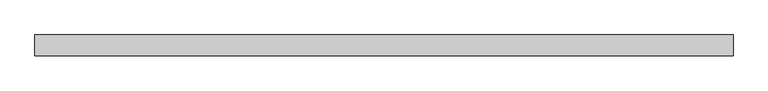
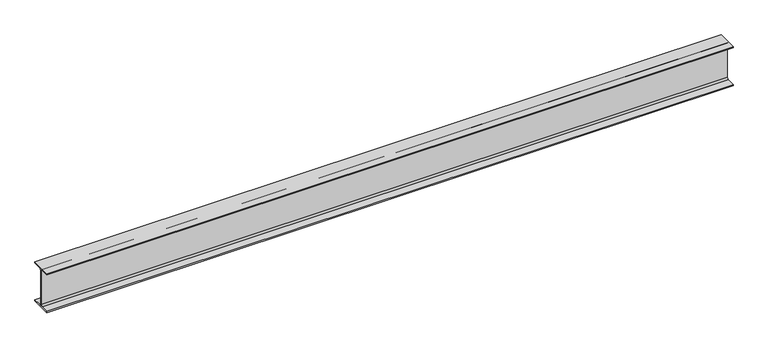
"""IFC4 building model written with IfcOpenShell, lengths in millimetres: beam geometry, 0912_Steel Framing_H-KSD3502 : H_SB_ASB_H-350x175x7x11."""

from ifc_helpers import new_model, si_unit, point, frame, frame_2d, origin, place, context, project, spatial, polyline, circle_curve, trimmed, segment, composite_curve, outline, extrude, source, transform, mapped, element, save


def beam_47c587fb(model_context):
    return source(origin(), model_context, "Body", "SweptSolid", [
        extrude(outline(composite_curve([segment(polyline([(87.5, -164.0), (87.5, -175.0), (-87.5, -175.0), (-87.5, -164.0), (-17.5, -164.0)]), True, "CONTINUOUS"), segment(trimmed(circle_curve(frame_2d((-17.5, -150.0)), 14.0), [point((-17.5, -164.0))], [point((-3.5, -150.0))], True, "CARTESIAN"), True, "CONTINUOUS"), segment(polyline([(-3.5, -150.0), (-3.5, 150.0)]), True, "CONTINUOUS"), segment(trimmed(circle_curve(frame_2d((-17.5, 150.0)), 14.0), [point((-3.5, 150.0))], [point((-17.5, 164.0))], True, "CARTESIAN"), True, "CONTINUOUS"), segment(polyline([(-17.5, 164.0), (-87.5, 164.0), (-87.5, 175.0), (87.5, 175.0), (87.5, 164.0), (17.5, 164.0)]), True, "CONTINUOUS"), segment(trimmed(circle_curve(frame_2d((17.5, 150.0)), 14.0), [point((17.5, 164.0))], [point((3.5, 150.0))], True, "CARTESIAN"), True, "CONTINUOUS"), segment(polyline([(3.5, 150.0), (3.5, -150.0)]), True, "CONTINUOUS"), segment(trimmed(circle_curve(frame_2d((17.5, -150.0)), 14.0), [point((3.5, -150.0))], [point((17.5, -164.0))], True, "CARTESIAN"), True, "CONTINUOUS"), segment(polyline([(17.5, -164.0), (87.5, -164.0)]), True, "CONTINUOUS")], self_intersect=False)), frame((-2914.177743, 0.0, 0.0), z_axis=(1.0, 0.0, 0.0), x_axis=(0.0, 1.0, 0.0)), (0.0, 0.0, 1.0), 5812.2452865),
    ])


if __name__ == "__main__":
    model = new_model("IFC4")
    model_context = context("Model", 3, world=origin())
    ifc_project = project(units=[si_unit("LENGTHUNIT", "METRE", prefix="MILLI")], contexts=[model_context])
    site = spatial("IfcSite", under=ifc_project)
    building = spatial("IfcBuilding", under=site)
    placement = place(None, origin())
    beam_shape = beam_47c587fb(model_context)
    element("IfcBeam", 1, ObjectType="0912_Steel Framing_H-KSD3502 : H_SB_ASB_H-350x175x7x11", at=placement, inside=building, context=model_context, shape_type="MappedRepresentation", body=[
        mapped(beam_shape, transform((0.0, 0.0, 0.0), x_axis=(1.0, 0.0, 0.0), y_axis=(0.0, 1.0, 0.0), z_axis=(0.0, 0.0, 1.0))),
    ])
    save(model, "model.ifc")

# Revit data of these elements
# Type "0912_Steel Framing_H-KSD3502 : H_SB_ASB_H-350x175x7x11"
#   H_WM Code_1 = "S01AA002-00001 | Main Steel Structure Fabrication Work | Shelter/Building | Medium Steel - Standard (90KG/M>Weight≥30KG/M) | Material: (   )"
#   H_WM Code_2 = "S03AA028-00001 | Main Steel Structure Erection Work | Shelter/Building | Medium Steel (90KG/M>Weight≥30KG/M) | Material: (   )"
#   H_WM Code_3 = "S01AA010-00001 | Main Steel Structure Fabrication Work | Shelter/Building | Steel Painting/Coating | for Non-Fireproofed Steel Surface, Surface Preparation, Primer, Second & Final Coat | Material: (   )"
#   H_Q'ty Cal Type Tag = "SB-Q2"
#   Width = 17.5 cm
#   Web Thickness = 0.7 cm
#   Web Fillet = 1.4 cm
#   Warping Constant = 282000.0 cm⁶
#   W = 0
#   Torsional Moment of Inertia = 19.4042 cm⁴
#   Section Area = 63.14 cm²
#   Plastic Modulus weak axis = 174.0 cm³
#   Plastic Modulus strong axis = 868.0 cm³
#   Perimeter = 1.36 m²/m
#   Nominal Weight = 49.60 kgf/m
#   Moment of Inertia weak axis = 984.00 cm⁴
#   Moment of Inertia strong axis = 13600.00 cm⁴
#   Height = 35.0 cm
#   Flange Thickness = 1.1 cm
#   Elastic Modulus weak axis = 112.0 cm³
#   Elastic Modulus strong axis = 775.0 cm³
#   Centroid Vertical = 17.5 cm
#   Centroid Horizontal = 8.75 cm
#   Ix = 136000000
#   Length [instance default] = 1.5240 m
#   Zx = 868000
#   b = 0.1750 m
#   h = 0.3500 m
#   r = 0.0140 m
#   s = 0.0070 m
#   t = 0.0110 m
#   A = 0.006314 m²
#   Structural Material [instance default] = Steel, 45-345
#   Assembly Code = ""
# Element 1 (IfcBeam, "0912_Steel Framing_H-KSD3502 : H_SB_ASB_H-350x175x7x11")
#   Structural Material = none
# Materials
#   "Steel, 45-345": class "Metal", colour RGB 189 187 185, transparency 0, Description = "Steel 345 MPa", Cost = 0
